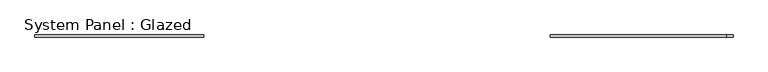
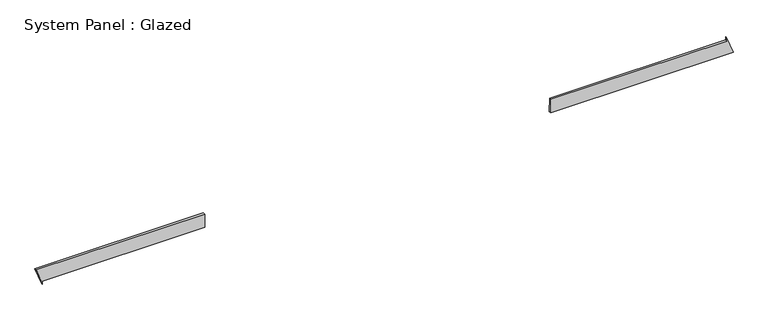
"""IFC4 building model written with IfcOpenShell, lengths in millimetres: plate geometry, System Panel : Glazed."""

import ifcopenshell
import ifcopenshell.guid

model = None  # the IFC model being written
_history = None  # IfcOwnerHistory: only IFC2X3 demands one
_inside = {}  # id of a spatial element -> (the spatial element, [elements in it])
_under = {}  # id of a project, library or spatial element -> (it, [spatial elements below it])
_declared = {}  # id of a project -> (the project, [libraries it declares])
_typed = {}  # id of a type object -> (the type object, [elements of that type])
_made_of = {}  # id of a material, layer set ... -> (it, [elements and type objects made of it])


def new_model(schema):
    """Start an empty IFC model of exactly this schema.

    Asked for "IFC4X3", IfcOpenShell would pick the latest addendum, in which some entities
    have other attributes; the version numbers below select the first issue.
    IFC2X3 requires an IfcOwnerHistory on every rooted entity: one is made here for all.
    """
    global model, _history
    if schema == "IFC4X3":
        model = ifcopenshell.file(schema_version=(4, 3, 0, 0))
    else:
        model = ifcopenshell.file(schema=schema)
    _inside.clear()
    _under.clear()
    _declared.clear()
    _typed.clear()
    _made_of.clear()
    _history = None
    if model.schema == "IFC2X3":
        org = make("IfcOrganization", Name="unknown")
        user = make(
            "IfcPersonAndOrganization",
            ThePerson=make("IfcPerson", FamilyName="unknown"),
            TheOrganization=org,
        )
        app = make(
            "IfcApplication",
            ApplicationDeveloper=org,
            Version="unknown",
            ApplicationFullName="unknown",
            ApplicationIdentifier="unknown",
        )
        _history = make(
            "IfcOwnerHistory",
            OwningUser=user,
            OwningApplication=app,
            ChangeAction="ADDED",
            CreationDate=0,
        )
    return model


def make(cls, **values):
    """One entity of the class cls with the attributes given. An attribute that is None is left unset."""
    return model.create_entity(
        cls, **{name: value for name, value in values.items() if value is not None}
    )


def rooted(cls, **values):
    """An entity with a GlobalId (a new one), such as an element, a storey or a relation."""
    return make(cls, GlobalId=ifcopenshell.guid.new(), OwnerHistory=_history, **values)


def si_unit(unit_type, name, prefix=None):
    """IfcSIUnit, for example si_unit("LENGTHUNIT", "METRE", prefix="MILLI")."""
    return make("IfcSIUnit", UnitType=unit_type, Prefix=prefix, Name=name)


def assignment(units):
    """IfcUnitAssignment: the units of a project."""
    return None if units is None else make("IfcUnitAssignment", Units=units)


def point(xyz):
    """IfcCartesianPoint."""
    return None if xyz is None else make("IfcCartesianPoint", Coordinates=xyz)


def direction(xyz):
    """IfcDirection."""
    return None if xyz is None else make("IfcDirection", DirectionRatios=xyz)


def frame(location, z_axis=None, x_axis=None):
    """IfcAxis2Placement3D, a coordinate frame: its origin and axes. An axis left out is left unset."""
    return make(
        "IfcAxis2Placement3D",
        Location=point(location),
        Axis=direction(z_axis),
        RefDirection=direction(x_axis),
    )


def origin():
    """The frame at (0, 0, 0) with its axes left unset."""
    return frame((0.0, 0.0, 0.0))


def place(relative_to, where):
    """IfcLocalPlacement: puts the frame where relative to a parent placement (None: the world)."""
    return make(
        "IfcLocalPlacement", PlacementRelTo=relative_to, RelativePlacement=where
    )


def context(
    kind, dimensions, precision=None, world=None, true_north=None, identifier=None
):
    """IfcGeometricRepresentationContext, for example the 3D "Model" context."""
    return make(
        "IfcGeometricRepresentationContext",
        ContextIdentifier=identifier,
        ContextType=kind,
        CoordinateSpaceDimension=dimensions,
        Precision=precision,
        WorldCoordinateSystem=world,
        TrueNorth=true_north,
    )


def project(units=None, contexts=None):
    """IfcProject with its units and contexts."""
    return rooted(
        "IfcProject",
        Name="project",
        RepresentationContexts=contexts,
        UnitsInContext=assignment(units),
    )


def spatial(cls, under=None, at=None, **own):
    """A site, building, storey or space (cls), placed at a placement, below another one or the project."""
    s = rooted(cls, ObjectPlacement=at, **own)
    if under is not None:
        _under.setdefault(under.id(), (under, []))[1].append(s)
    return s


def polyline(points):
    """IfcPolyline through the points."""
    return make("IfcPolyline", Points=[point(p) for p in points])


def outline(outer, holes=None, kind="AREA"):
    """IfcArbitraryClosedProfileDef: a profile drawn as a closed curve; with holes, ...WithVoids."""
    if holes is None:
        return make("IfcArbitraryClosedProfileDef", ProfileType=kind, OuterCurve=outer)
    return make(
        "IfcArbitraryProfileDefWithVoids",
        ProfileType=kind,
        OuterCurve=outer,
        InnerCurves=holes,
    )


def extrude(swept, where, along, depth):
    """IfcExtrudedAreaSolid: the profile swept, set in the frame where, extruded along a direction by depth."""
    return make(
        "IfcExtrudedAreaSolid",
        SweptArea=swept,
        Position=where,
        ExtrudedDirection=direction(along),
        Depth=depth,
    )


def shape(context_of_items, identifier, shape_type, items):
    """IfcShapeRepresentation: the items that make up one representation, for example the "Body"."""
    return make(
        "IfcShapeRepresentation",
        ContextOfItems=context_of_items,
        RepresentationIdentifier=identifier,
        RepresentationType=shape_type,
        Items=items,
    )


def source(mapping_origin, context_of_items, identifier, shape_type, items):
    """IfcRepresentationMap: a shape defined once, which mapped items show again and again."""
    return make(
        "IfcRepresentationMap",
        MappingOrigin=mapping_origin,
        MappedRepresentation=shape(context_of_items, identifier, shape_type, items),
    )


def transform(
    local_origin,
    x_axis=None,
    y_axis=None,
    z_axis=None,
    scale=None,
    scale2=None,
    scale3=None,
    uniform=True,
):
    """IfcCartesianTransformationOperator3D, or its non-uniform kind. x_axis, y_axis, z_axis: its Axis1, 2, 3."""
    if uniform:
        return make(
            "IfcCartesianTransformationOperator3D",
            Axis1=direction(x_axis),
            Axis2=direction(y_axis),
            LocalOrigin=point(local_origin),
            Scale=scale,
            Axis3=direction(z_axis),
        )
    return make(
        "IfcCartesianTransformationOperator3DnonUniform",
        Axis1=direction(x_axis),
        Axis2=direction(y_axis),
        LocalOrigin=point(local_origin),
        Scale=scale,
        Axis3=direction(z_axis),
        Scale2=scale2,
        Scale3=scale3,
    )


def mapped(mapping_source, mapping_target):
    """IfcMappedItem: shows the shape of a source again, moved by a transform."""
    return make(
        "IfcMappedItem", MappingSource=mapping_source, MappingTarget=mapping_target
    )


def made_of(thing, what):
    """Note that an element or type object is made of a material, layer set ...; save() writes the relation."""
    if what is not None:
        _made_of.setdefault(what.id(), (what, []))[1].append(thing)
    return thing


def element(
    cls,
    number,
    at=None,
    inside=None,
    cuts=None,
    type_object=None,
    material=None,
    context=None,
    identifier="Body",
    shape_type=None,
    held_by="IfcProductDefinitionShape",
    body=None,
    shapes=None,
    **own,
):
    """One element of the class cls, such as IfcWall. Its Tag is "e" and its number.

    at: its placement. inside: the storey or other place that contains it. cuts: it is an
    opening in that element (IfcRelVoidsElement). A single representation is given by context,
    identifier, shape_type and body (its items); several are given by shapes. held_by: the class
    of the entity that holds the representations. save() writes the other relations.
    """
    e = rooted(cls, Tag="e%d" % number, ObjectPlacement=at, **own)
    if body is not None:
        shapes = [shape(context, identifier, shape_type, body)]
    if shapes is not None:
        e.Representation = make(held_by, Representations=shapes)
    if inside is not None:
        _inside.setdefault(inside.id(), (inside, []))[1].append(e)
    if cuts is not None:
        rooted(
            "IfcRelVoidsElement", RelatingBuildingElement=cuts, RelatedOpeningElement=e
        )
    if type_object is not None:
        _typed.setdefault(type_object.id(), (type_object, []))[1].append(e)
    return made_of(e, material)


def aggregate(whole, parts):
    """IfcRelAggregates: a whole, such as a stair, and the parts it consists of."""
    return rooted("IfcRelAggregates", RelatingObject=whole, RelatedObjects=parts)


def save(model, path):
    """Write the relations noted so far, then the file.

    IfcRelAggregates (storeys below a building ...), IfcRelContainedInSpatialStructure (elements
    in a storey), IfcRelDefinesByType, IfcRelAssociatesMaterial and IfcRelDeclares: one each for
    every whole, place, type object, material and project.
    """
    for whole, parts in _under.values():
        aggregate(whole, parts)
    for where, things in _inside.values():
        rooted(
            "IfcRelContainedInSpatialStructure",
            RelatedElements=things,
            RelatingStructure=where,
        )
    for kind, things in _typed.values():
        rooted("IfcRelDefinesByType", RelatedObjects=things, RelatingType=kind)
    for what, things in _made_of.values():
        rooted("IfcRelAssociatesMaterial", RelatedObjects=things, RelatingMaterial=what)
    for by, libraries in _declared.values():
        rooted("IfcRelDeclares", RelatingContext=by, RelatedDefinitions=libraries)
    model.write(path)


def system_panel_glazed_641e3d16(model_context):
    return source(origin(), model_context, "Body", "SweptSolid", [
        extrude(outline(polyline([(0.0, -3957.2941299), (35.3553391, -3957.2941299), (35.3553391, -2080.9817209), (198.4286437, -2081.9508043), (198.5124481, -4028.0649835), (0.0, -3957.2941299)])), frame((0.0, -49.5, 0.0), z_axis=(0.0, 1.0, 0.0), x_axis=(0.0, 0.0, 1.0)), (0.0, 0.0, 1.0), 25.0),
        extrude(outline(polyline([(35.3553391, 1920.0844805), (35.3553391, 4028.0649835), (233.5239524, 3956.4980838), (198.1686134, 3956.4965613), (198.2562684, 1920.9642368), (35.3553391, 1920.0844805)])), frame((0.0, -49.5, 0.0), z_axis=(0.0, 1.0, 0.0), x_axis=(0.0, 0.0, 1.0)), (0.0, 0.0, 1.0), 25.0),
    ])


if __name__ == "__main__":
    model = new_model("IFC4")
    model_context = context("Model", 3, world=origin())
    ifc_project = project(units=[si_unit("LENGTHUNIT", "METRE", prefix="MILLI")], contexts=[model_context])
    site = spatial("IfcSite", under=ifc_project)
    building = spatial("IfcBuilding", under=site)
    placement = place(None, origin())
    system_panel_glazed_shape = system_panel_glazed_641e3d16(model_context)
    element("IfcPlate", 1, ObjectType="System Panel : Glazed", at=placement, inside=building, context=model_context, shape_type="MappedRepresentation", body=[
        mapped(system_panel_glazed_shape, transform((0.0, 0.0, 0.0), x_axis=(1.0, 0.0, 0.0), y_axis=(0.0, 1.0, 0.0), z_axis=(0.0, 0.0, 1.0))),
    ])
    save(model, "model.ifc")

# Revit data of these elements
# Element 1 (IfcPlate, "System Panel : Glazed")
#   Materials on its faces: "Glass"
# Materials
#   "Glass": class "Glass", colour RGB 218 227 224, transparency 0.85, Description = "Soda Lime Glass", Cost = 0
